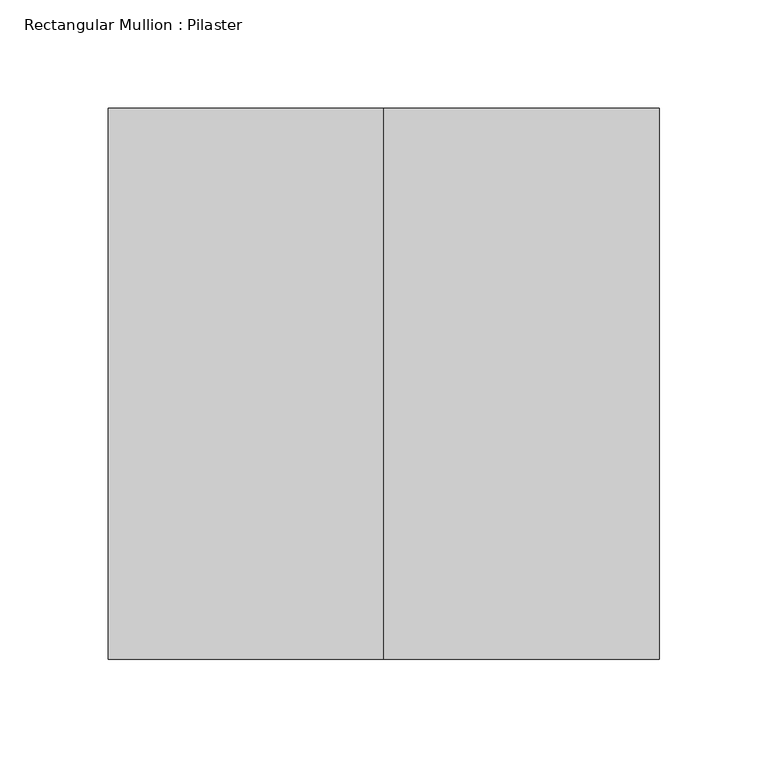
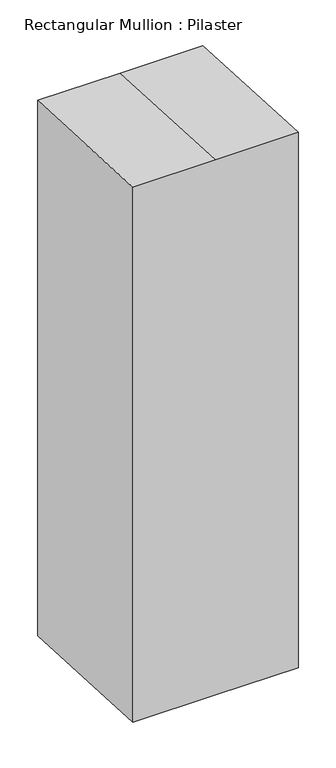
"""IFC4 building model written with IfcOpenShell, lengths in millimetres: member geometry, Rectangular Mullion : Pilaster."""

from ifc_helpers import new_model, si_unit, origin, place, context, project, spatial, faceted_brep, source, transform, mapped, element, save


def rectangular_mullion_pilaster_fddbf53e(model_context):
    return source(origin(), model_context, "Body", "Brep", [
        faceted_brep([(-127.0, 127.0, -2.7320304), (0.0, 127.0, -2.7320304), (127.0, 127.0, -2.7320304), (127.0, 127.0, -872.2393518), (0.0, 127.0, -872.2393518), (-127.0, 127.0, -872.2393518), (-127.0, -127.0, 10.5795456), (-127.0, -127.0, -858.9277759), (127.0, -127.0, 10.5795456), (0.0, -127.0, 10.5795456), (0.0, -127.0, -858.9277759), (127.0, -127.0, -858.9277759)], [[[0, 1, 2, 3, 4, 5]], [[6, 0, 5, 7]], [[8, 9, 6, 7, 10, 11]], [[2, 8, 11, 3]], [[2, 1, 9, 8]], [[1, 0, 6, 9]], [[3, 11, 10, 4]], [[10, 7, 5, 4]]]),
    ])


if __name__ == "__main__":
    model = new_model("IFC4")
    model_context = context("Model", 3, world=origin())
    ifc_project = project(units=[si_unit("LENGTHUNIT", "METRE", prefix="MILLI")], contexts=[model_context])
    site = spatial("IfcSite", under=ifc_project)
    building = spatial("IfcBuilding", under=site)
    placement = place(None, origin())
    rectangular_mullion_pilaster_shape = rectangular_mullion_pilaster_fddbf53e(model_context)
    element("IfcMember", 1, ObjectType="Rectangular Mullion : Pilaster", at=placement, inside=building, context=model_context, shape_type="MappedRepresentation", body=[
        mapped(rectangular_mullion_pilaster_shape, transform((0.0, 0.0, 0.0), x_axis=(1.0, 0.0, 0.0), y_axis=(0.0, 1.0, 0.0), z_axis=(0.0, 0.0, 1.0))),
    ])
    save(model, "model.ifc")

# Revit data of these elements
# Type "Rectangular Mullion : Pilaster"
#   built-in parameter 1007304 = 0.833333 (stored number, unit not read)
#   built-in parameter 1007301 = 0.416667 (stored number, unit not read)
#   built-in parameter 1007300 = 0.416667 (stored number, unit not read)
# Element 1 (IfcMember, "Rectangular Mullion : Pilaster")
#   Materials on its faces: "Aluminum"
# Materials
#   "Aluminum": class "Metal", colour RGB 247 247 247, transparency 0, Description = "Aluminum 6061", Cost = 0
